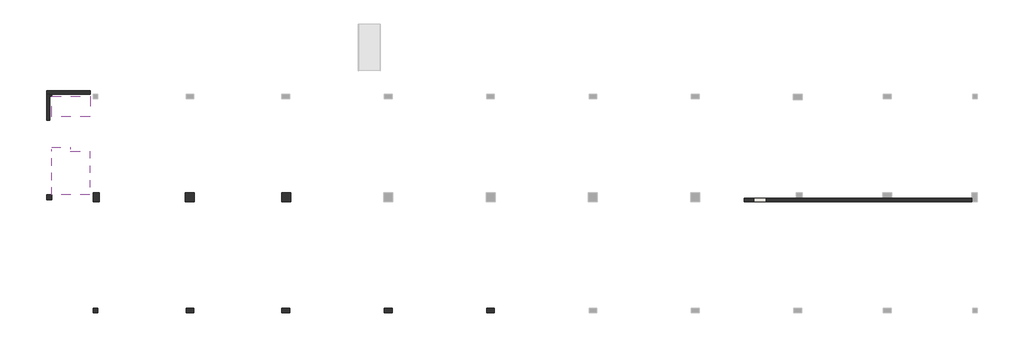
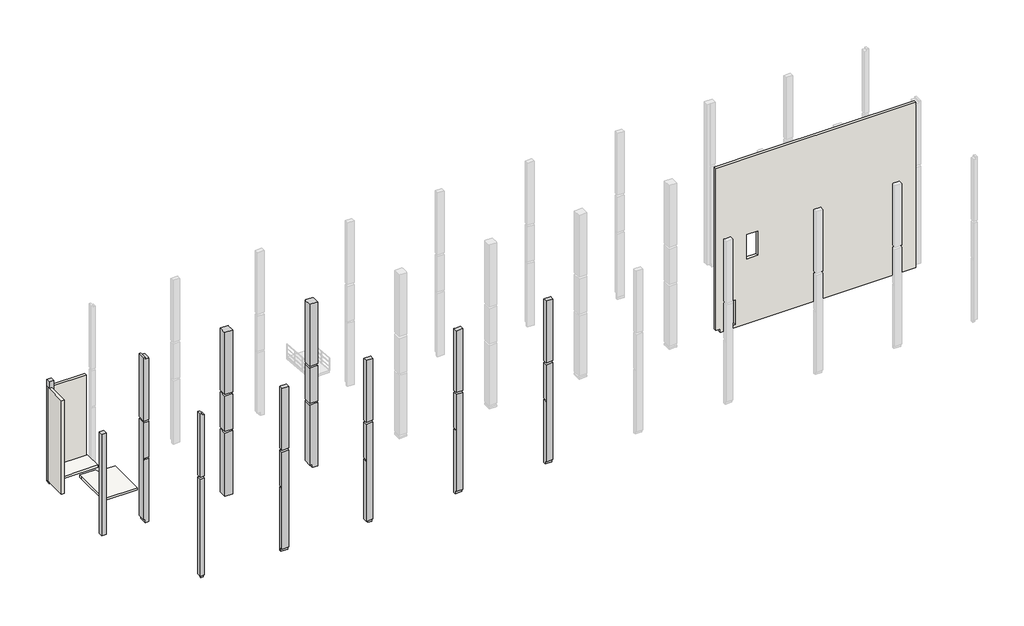
# One storey, part 1 of 3: 10 columns, 3 walls, 2 slabs.
"""IFC4 building model written with IfcOpenShell, lengths in millimetres."""

import ifcopenshell
import ifcopenshell.guid

model = None  # the IFC model being written
_history = None  # IfcOwnerHistory: only IFC2X3 demands one
_inside = {}  # id of a spatial element -> (the spatial element, [elements in it])
_under = {}  # id of a project, library or spatial element -> (it, [spatial elements below it])
_declared = {}  # id of a project -> (the project, [libraries it declares])
_typed = {}  # id of a type object -> (the type object, [elements of that type])
_made_of = {}  # id of a material, layer set ... -> (it, [elements and type objects made of it])


def new_model(schema):
    """Start an empty IFC model of exactly this schema.

    Asked for "IFC4X3", IfcOpenShell would pick the latest addendum, in which some entities
    have other attributes; the version numbers below select the first issue.
    IFC2X3 requires an IfcOwnerHistory on every rooted entity: one is made here for all.
    """
    global model, _history
    if schema == "IFC4X3":
        model = ifcopenshell.file(schema_version=(4, 3, 0, 0))
    else:
        model = ifcopenshell.file(schema=schema)
    _inside.clear()
    _under.clear()
    _declared.clear()
    _typed.clear()
    _made_of.clear()
    _history = None
    if model.schema == "IFC2X3":
        org = make("IfcOrganization", Name="unknown")
        user = make(
            "IfcPersonAndOrganization",
            ThePerson=make("IfcPerson", FamilyName="unknown"),
            TheOrganization=org,
        )
        app = make(
            "IfcApplication",
            ApplicationDeveloper=org,
            Version="unknown",
            ApplicationFullName="unknown",
            ApplicationIdentifier="unknown",
        )
        _history = make(
            "IfcOwnerHistory",
            OwningUser=user,
            OwningApplication=app,
            ChangeAction="ADDED",
            CreationDate=0,
        )
    return model


def make(cls, **values):
    """One entity of the class cls with the attributes given. An attribute that is None is left unset."""
    return model.create_entity(
        cls, **{name: value for name, value in values.items() if value is not None}
    )


def rooted(cls, **values):
    """An entity with a GlobalId (a new one), such as an element, a storey or a relation."""
    return make(cls, GlobalId=ifcopenshell.guid.new(), OwnerHistory=_history, **values)


def si_unit(unit_type, name, prefix=None):
    """IfcSIUnit, for example si_unit("LENGTHUNIT", "METRE", prefix="MILLI")."""
    return make("IfcSIUnit", UnitType=unit_type, Prefix=prefix, Name=name)


def assignment(units):
    """IfcUnitAssignment: the units of a project."""
    return None if units is None else make("IfcUnitAssignment", Units=units)


def point(xyz):
    """IfcCartesianPoint."""
    return None if xyz is None else make("IfcCartesianPoint", Coordinates=xyz)


def direction(xyz):
    """IfcDirection."""
    return None if xyz is None else make("IfcDirection", DirectionRatios=xyz)


def frame(location, z_axis=None, x_axis=None):
    """IfcAxis2Placement3D, a coordinate frame: its origin and axes. An axis left out is left unset."""
    return make(
        "IfcAxis2Placement3D",
        Location=point(location),
        Axis=direction(z_axis),
        RefDirection=direction(x_axis),
    )


def origin():
    """The frame at (0, 0, 0) with its axes left unset."""
    return frame((0.0, 0.0, 0.0))


def place(relative_to, where):
    """IfcLocalPlacement: puts the frame where relative to a parent placement (None: the world)."""
    return make(
        "IfcLocalPlacement", PlacementRelTo=relative_to, RelativePlacement=where
    )


def context(
    kind, dimensions, precision=None, world=None, true_north=None, identifier=None
):
    """IfcGeometricRepresentationContext, for example the 3D "Model" context."""
    return make(
        "IfcGeometricRepresentationContext",
        ContextIdentifier=identifier,
        ContextType=kind,
        CoordinateSpaceDimension=dimensions,
        Precision=precision,
        WorldCoordinateSystem=world,
        TrueNorth=true_north,
    )


def project(units=None, contexts=None):
    """IfcProject with its units and contexts."""
    return rooted(
        "IfcProject",
        Name="project",
        RepresentationContexts=contexts,
        UnitsInContext=assignment(units),
    )


def spatial(cls, under=None, at=None, **own):
    """A site, building, storey or space (cls), placed at a placement, below another one or the project."""
    s = rooted(cls, ObjectPlacement=at, **own)
    if under is not None:
        _under.setdefault(under.id(), (under, []))[1].append(s)
    return s


def polyline(points):
    """IfcPolyline through the points."""
    return make("IfcPolyline", Points=[point(p) for p in points])


def outline(outer, holes=None, kind="AREA"):
    """IfcArbitraryClosedProfileDef: a profile drawn as a closed curve; with holes, ...WithVoids."""
    if holes is None:
        return make("IfcArbitraryClosedProfileDef", ProfileType=kind, OuterCurve=outer)
    return make(
        "IfcArbitraryProfileDefWithVoids",
        ProfileType=kind,
        OuterCurve=outer,
        InnerCurves=holes,
    )


def extrude(swept, where, along, depth):
    """IfcExtrudedAreaSolid: the profile swept, set in the frame where, extruded along a direction by depth."""
    return make(
        "IfcExtrudedAreaSolid",
        SweptArea=swept,
        Position=where,
        ExtrudedDirection=direction(along),
        Depth=depth,
    )


def faces_of(points, faces, orient=None, outer=None):
    """IfcFace entities. A face is a list of loops; a loop is a list of indices into points, from 0.

    orient and outer hold one flag for each loop. By default every Orientation is true, the
    first loop of a face is its IfcFaceOuterBound and the others are IfcFaceBound.
    """
    made = []
    for i, loops in enumerate(faces):
        bounds = []
        for j, loop in enumerate(loops):
            is_outer = j == 0 if outer is None else outer[i][j]
            bounds.append(
                make(
                    "IfcFaceOuterBound" if is_outer else "IfcFaceBound",
                    Bound=make("IfcPolyLoop", Polygon=[points[k] for k in loop]),
                    Orientation=True if orient is None else orient[i][j],
                )
            )
        made.append(make("IfcFace", Bounds=bounds))
    return made


def faceted_brep(points, faces, orient=None, outer=None, voids=None):
    """IfcFacetedBrep: a solid bounded by flat faces; with voids (closed shells), ...WithVoids."""
    shared = [point(p) for p in points]
    hull = make("IfcClosedShell", CfsFaces=faces_of(shared, faces, orient, outer))
    if voids is None:
        return make("IfcFacetedBrep", Outer=hull)
    return make(
        "IfcFacetedBrepWithVoids",
        Outer=hull,
        Voids=[
            make(cls, CfsFaces=faces_of(shared, fs, o, b)) for cls, fs, o, b in voids
        ],
    )


def shape(context_of_items, identifier, shape_type, items):
    """IfcShapeRepresentation: the items that make up one representation, for example the "Body"."""
    return make(
        "IfcShapeRepresentation",
        ContextOfItems=context_of_items,
        RepresentationIdentifier=identifier,
        RepresentationType=shape_type,
        Items=items,
    )


def made_of(thing, what):
    """Note that an element or type object is made of a material, layer set ...; save() writes the relation."""
    if what is not None:
        _made_of.setdefault(what.id(), (what, []))[1].append(thing)
    return thing


def element(
    cls,
    number,
    at=None,
    inside=None,
    cuts=None,
    type_object=None,
    material=None,
    context=None,
    identifier="Body",
    shape_type=None,
    held_by="IfcProductDefinitionShape",
    body=None,
    shapes=None,
    **own,
):
    """One element of the class cls, such as IfcWall. Its Tag is "e" and its number.

    at: its placement. inside: the storey or other place that contains it. cuts: it is an
    opening in that element (IfcRelVoidsElement). A single representation is given by context,
    identifier, shape_type and body (its items); several are given by shapes. held_by: the class
    of the entity that holds the representations. save() writes the other relations.
    """
    e = rooted(cls, Tag="e%d" % number, ObjectPlacement=at, **own)
    if body is not None:
        shapes = [shape(context, identifier, shape_type, body)]
    if shapes is not None:
        e.Representation = make(held_by, Representations=shapes)
    if inside is not None:
        _inside.setdefault(inside.id(), (inside, []))[1].append(e)
    if cuts is not None:
        rooted(
            "IfcRelVoidsElement", RelatingBuildingElement=cuts, RelatedOpeningElement=e
        )
    if type_object is not None:
        _typed.setdefault(type_object.id(), (type_object, []))[1].append(e)
    return made_of(e, material)


def aggregate(whole, parts):
    """IfcRelAggregates: a whole, such as a stair, and the parts it consists of."""
    return rooted("IfcRelAggregates", RelatingObject=whole, RelatedObjects=parts)


def save(model, path):
    """Write the relations noted so far, then the file.

    IfcRelAggregates (storeys below a building ...), IfcRelContainedInSpatialStructure (elements
    in a storey), IfcRelDefinesByType, IfcRelAssociatesMaterial and IfcRelDeclares: one each for
    every whole, place, type object, material and project.
    """
    for whole, parts in _under.values():
        aggregate(whole, parts)
    for where, things in _inside.values():
        rooted(
            "IfcRelContainedInSpatialStructure",
            RelatedElements=things,
            RelatingStructure=where,
        )
    for kind, things in _typed.values():
        rooted("IfcRelDefinesByType", RelatedObjects=things, RelatingType=kind)
    for what, things in _made_of.values():
        rooted("IfcRelAssociatesMaterial", RelatedObjects=things, RelatingMaterial=what)
    for by, libraries in _declared.values():
        rooted("IfcRelDeclares", RelatingContext=by, RelatedDefinitions=libraries)
    model.write(path)


model = new_model("IFC4")

# Units and contexts
model_context = context("Model", 3, world=origin())
ifc_project = project(units=[si_unit("LENGTHUNIT", "METRE", prefix="MILLI")], contexts=[model_context])

# Site, building, storey
site = spatial("IfcSite", under=ifc_project)
building = spatial("IfcBuilding", under=site)
storey = spatial("IfcBuildingStorey", under=building, Name="G.L", Elevation=-150.0381366)

# Columns
placement = place(None, origin())
element("IfcColumn", 1, ObjectType="RC_Column_Rectangular : H_SC_AR_S15_AG_W700xL700_C1", at=placement, inside=storey, context=model_context, shape_type="Brep", body=[
    faceted_brep([(400.0, 9849.5208589, -150.0381366), (400.0, 9149.5208589, -150.0381366), (100.0, 9149.5208589, -150.0381366), (100.0, 9849.5208589, -150.0381366), (0.0, 9849.5208589, 5799.9618634), (0.0, 9149.5208589, 5799.9618634), (100.0, 9149.5208589, 5799.9618634), (400.0, 9149.5208589, 5799.9618634), (400.0, 9199.5208589, 5799.9618634), (400.0, 9799.5208589, 5799.9618634), (400.0, 9849.5208589, 5799.9618634), (150.0, 9849.5208589, 5799.9618634), (100.0, 9849.5208589, 5799.9618634), (0.0, 9149.5208589, 5949.9618634), (0.0, 9849.5208589, 5949.9618634), (400.0, 9849.5208589, 5949.9618634), (400.0, 9149.5208589, 5949.9618634), (0.0, 9849.5208589, 5899.9618634), (400.0, 9149.5208589, 9269.9618634), (400.0, 9199.5208589, 9269.9618634), (400.0, 9799.5208589, 9269.9618634), (400.0, 9849.5208589, 9269.9618634), (100.0, 9849.5208589, 9269.9618634), (-50.0, 9849.5208589, 9269.9618634), (-50.0, 9149.5208589, 9269.9618634), (100.0, 9149.5208589, 9269.9618634), (100.0, 9149.5208589, 149.9618634), (100.0, 9849.5208589, 149.9618634), (-50.0, 9149.5208589, 149.9618634), (-50.0, 9849.5208589, 149.9618634), (-50.0, 9149.5208589, 5249.9618634), (-50.0, 9149.5208589, 5949.9618634), (-50.0, 9149.5208589, 8749.9618634), (-50.0, 9849.5208589, 8749.9618634), (-50.0, 9849.5208589, 5949.9618634), (-50.0, 9849.5208589, 5899.9618634), (-50.0, 9849.5208589, 5199.9618634)], [[[0, 1, 2, 3]], [[4, 5, 6, 7, 8, 9, 10, 11, 12]], [[13, 14, 15, 16]], [[5, 4, 17, 14, 13]], [[1, 0, 10, 9, 8, 7]], [[18, 19, 20, 21, 22, 23, 24, 25]], [[16, 15, 21, 20, 19, 18]], [[26, 27, 3, 2]], [[27, 26, 28, 29]], [[28, 30, 31, 32, 24, 23, 33, 34, 35, 36, 29]], [[1, 7, 6, 5, 13, 16, 18, 25, 24, 32, 31, 30, 28, 26, 2]], [[10, 0, 3, 27, 29, 36, 35, 34, 33, 23, 22, 21, 15, 14, 17, 4, 12, 11]]]),
    faceted_brep([(400.0, 9149.5208589, 9449.9618634), (400.0, 9849.5208589, 9449.9618634), (400.0, 9849.5208589, 15259.9618634), (400.0, 9724.5208589, 15259.9618634), (400.0, 9274.5208589, 15259.9618634), (400.0, 9149.5208589, 15259.9618634), (-50.0, 9149.5208589, 9449.9618634), (100.0, 9149.5208589, 15259.9618634), (100.0, 9149.5208589, 15409.9618634), (-50.0, 9149.5208589, 15409.9618634), (-50.0, 9149.5208589, 14709.9618634), (-50.0, 9849.5208589, 9449.9618634), (-50.0, 9849.5208589, 14709.9618634), (-50.0, 9849.5208589, 15409.9618634), (100.0, 9849.5208589, 15409.9618634), (100.0, 9849.5208589, 15259.9618634)], [[[0, 1, 2, 3, 4, 5]], [[6, 0, 5, 7, 8, 9, 10]], [[1, 11, 12, 13, 14, 15, 2]], [[8, 14, 13, 9]], [[1, 0, 6, 11]], [[15, 7, 5, 4, 3, 2]], [[7, 15, 14, 8]], [[6, 10, 9, 13, 12, 11]]]),
])
element("IfcColumn", 2, ObjectType="RC_Column_Rectangular : H_SC_AR_S15_AG_W700xL700_C1", at=placement, inside=storey, context=model_context, shape_type="Brep", body=[
    faceted_brep([(7850.0, 9849.5208589, -150.0381366), (7850.0, 9149.5208589, -150.0381366), (7150.0, 9149.5208589, -150.0381366), (7150.0, 9849.5208589, -150.0381366), (7850.0, 9149.5208589, 5799.9618634), (7850.0, 9199.5208589, 5799.9618634), (7850.0, 9799.5208589, 5799.9618634), (7850.0, 9849.5208589, 5799.9618634), (7750.0, 9849.5208589, 5799.9618634), (7250.0, 9849.5208589, 5799.9618634), (7150.0, 9849.5208589, 5799.9618634), (7150.0, 9799.5208589, 5799.9618634), (7150.0, 9199.5208589, 5799.9618634), (7150.0, 9149.5208589, 5799.9618634), (7250.0, 9149.5208589, 5799.9618634), (7750.0, 9149.5208589, 5799.9618634)], [[[0, 1, 2, 3]], [[4, 5, 6, 7, 8, 9, 10, 11, 12, 13, 14, 15]], [[1, 0, 7, 6, 5, 4]], [[2, 1, 4, 15, 14, 13]], [[3, 2, 13, 12, 11, 10]], [[0, 3, 10, 9, 8, 7]]]),
    faceted_brep([(7850.0, 9149.5208589, 9449.9618634), (7850.0, 9849.5208589, 9449.9618634), (7850.0, 9849.5208589, 15259.9618634), (7850.0, 9724.5208589, 15259.9618634), (7850.0, 9274.5208589, 15259.9618634), (7850.0, 9149.5208589, 15259.9618634), (7150.0, 9149.5208589, 9449.9618634), (7725.0, 9149.5208589, 15259.9618634), (7275.0, 9149.5208589, 15259.9618634), (7150.0, 9149.5208589, 15259.9618634), (7150.0, 9849.5208589, 9449.9618634), (7150.0, 9274.5208589, 15259.9618634), (7150.0, 9724.5208589, 15259.9618634), (7150.0, 9849.5208589, 15259.9618634), (7275.0, 9849.5208589, 15259.9618634), (7725.0, 9849.5208589, 15259.9618634)], [[[0, 1, 2, 3, 4, 5]], [[6, 0, 5, 7, 8, 9]], [[10, 6, 9, 11, 12, 13]], [[1, 10, 13, 14, 15, 2]], [[1, 0, 6, 10]], [[5, 4, 3, 2, 15, 14, 13, 12, 11, 9, 8, 7]]]),
    faceted_brep([(7850.0, 9849.5208589, 5949.9618634), (7850.0, 9149.5208589, 5949.9618634), (7150.0, 9149.5208589, 5949.9618634), (7150.0, 9849.5208589, 5949.9618634), (7850.0, 9149.5208589, 9269.9618634), (7850.0, 9199.5208589, 9269.9618634), (7850.0, 9799.5208589, 9269.9618634), (7850.0, 9849.5208589, 9269.9618634), (7750.0, 9849.5208589, 9269.9618634), (7250.0, 9849.5208589, 9269.9618634), (7150.0, 9849.5208589, 9269.9618634), (7150.0, 9799.5208589, 9269.9618634), (7150.0, 9199.5208589, 9269.9618634), (7150.0, 9149.5208589, 9269.9618634), (7250.0, 9149.5208589, 9269.9618634), (7750.0, 9149.5208589, 9269.9618634)], [[[0, 1, 2, 3]], [[4, 5, 6, 7, 8, 9, 10, 11, 12, 13, 14, 15]], [[1, 0, 7, 6, 5, 4]], [[2, 1, 4, 15, 14, 13]], [[3, 2, 13, 12, 11, 10]], [[0, 3, 10, 9, 8, 7]]]),
])
element("IfcColumn", 3, ObjectType="RC_Column_Rectangular : H_SC_AR_S15_AG_W700xL700_C1", at=placement, inside=storey, context=model_context, shape_type="Brep", body=[
    faceted_brep([(15400.0, 9849.5208589, -150.0381366), (15400.0, 9149.5208589, -150.0381366), (14950.0, 9149.5208589, -150.0381366), (14950.0, 9849.5208589, -150.0381366), (15400.0, 9149.5208589, 5799.9618634), (15400.0, 9199.5208589, 5799.9618634), (15400.0, 9799.5208589, 5799.9618634), (15400.0, 9849.5208589, 5799.9618634), (15250.0, 9849.5208589, 5799.9618634), (14750.0, 9849.5208589, 5799.9618634), (14700.0, 9849.5208589, 5799.9618634), (14700.0, 9799.5208589, 5799.9618634), (14700.0, 9199.5208589, 5799.9618634), (14700.0, 9149.5208589, 5799.9618634), (14750.0, 9149.5208589, 5799.9618634), (15250.0, 9149.5208589, 5799.9618634), (15400.0, 9849.5208589, -0.0381366), (15400.0, 9849.5208589, 149.9618634), (15400.0, 9149.5208589, 149.9618634), (15400.0, 9149.5208589, -0.0381366), (14700.0, 9149.5208589, 149.9618634), (14950.0, 9149.5208589, 149.9618634), (14950.0, 9149.5208589, -0.0381366), (14700.0, 9849.5208589, 149.9618634), (14950.0, 9849.5208589, -0.0381366), (14950.0, 9849.5208589, 149.9618634)], [[[0, 1, 2, 3]], [[4, 5, 6, 7, 8, 9, 10, 11, 12, 13, 14, 15]], [[1, 0, 16, 17, 7, 6, 5, 4, 18, 19]], [[1, 19, 18, 4, 15, 14, 13, 20, 21, 22, 2]], [[13, 12, 11, 10, 23, 20]], [[16, 0, 3, 24, 25, 23, 10, 9, 8, 7, 17]], [[21, 25, 24, 3, 2, 22]], [[25, 21, 20, 23]]]),
    faceted_brep([(15400.0, 9149.5208589, 9449.9618634), (15400.0, 9849.5208589, 9449.9618634), (15400.0, 9849.5208589, 15259.9618634), (15400.0, 9724.5208589, 15259.9618634), (15400.0, 9274.5208589, 15259.9618634), (15400.0, 9149.5208589, 15259.9618634), (14700.0, 9149.5208589, 9449.9618634), (15225.0, 9149.5208589, 15259.9618634), (14775.0, 9149.5208589, 15259.9618634), (14700.0, 9149.5208589, 15259.9618634), (14700.0, 9849.5208589, 9449.9618634), (14700.0, 9274.5208589, 15259.9618634), (14700.0, 9724.5208589, 15259.9618634), (14700.0, 9849.5208589, 15259.9618634), (14775.0, 9849.5208589, 15259.9618634), (15225.0, 9849.5208589, 15259.9618634)], [[[0, 1, 2, 3, 4, 5]], [[6, 0, 5, 7, 8, 9]], [[10, 6, 9, 11, 12, 13]], [[1, 10, 13, 14, 15, 2]], [[1, 0, 6, 10]], [[5, 4, 3, 2, 15, 14, 13, 12, 11, 9, 8, 7]]]),
    faceted_brep([(15400.0, 9849.5208589, 5949.9618634), (15400.0, 9149.5208589, 5949.9618634), (14700.0, 9149.5208589, 5949.9618634), (14700.0, 9849.5208589, 5949.9618634), (15400.0, 9149.5208589, 9269.9618634), (15400.0, 9199.5208589, 9269.9618634), (15400.0, 9799.5208589, 9269.9618634), (15400.0, 9849.5208589, 9269.9618634), (15250.0, 9849.5208589, 9269.9618634), (14750.0, 9849.5208589, 9269.9618634), (14700.0, 9849.5208589, 9269.9618634), (14700.0, 9799.5208589, 9269.9618634), (14700.0, 9199.5208589, 9269.9618634), (14700.0, 9149.5208589, 9269.9618634), (14750.0, 9149.5208589, 9269.9618634), (15250.0, 9149.5208589, 9269.9618634)], [[[0, 1, 2, 3]], [[4, 5, 6, 7, 8, 9, 10, 11, 12, 13, 14, 15]], [[1, 0, 7, 6, 5, 4]], [[2, 1, 4, 15, 14, 13]], [[3, 2, 13, 12, 11, 10]], [[0, 3, 10, 9, 8, 7]]]),
])
element("IfcColumn", 4, ObjectType="RC_Column_Rectangular : H_SC_AR_S15_AG_W600xL600_C2", at=placement, inside=storey, context=model_context, shape_type="Brep", body=[
    faceted_brep([(30700.0, 799.5208589, -150.0381366), (31300.0, 799.5208589, -150.0381366), (31300.0, 599.5208589, -150.0381366), (30700.0, 599.5208589, -150.0381366), (30700.0, 499.5208589, 5799.9618634), (31300.0, 499.5208589, 5799.9618634), (31300.0, 599.5208589, 5799.9618634), (31300.0, 799.5208589, 5799.9618634), (31250.0, 799.5208589, 5799.9618634), (30750.0, 799.5208589, 5799.9618634), (30700.0, 799.5208589, 5799.9618634), (30700.0, 599.5208589, 5799.9618634), (31300.0, 499.5208589, 5949.9618634), (30700.0, 499.5208589, 5949.9618634), (30700.0, 799.5208589, 5949.9618634), (31300.0, 799.5208589, 5949.9618634), (30700.0, 799.5208589, -0.0381366), (30700.0, 799.5208589, 149.9618634), (31300.0, 799.5208589, 149.9618634), (31300.0, 799.5208589, -0.0381366), (31300.0, 449.5208589, 9269.9618634), (31300.0, 599.5208589, 9269.9618634), (31300.0, 799.5208589, 9269.9618634), (31250.0, 799.5208589, 9269.9618634), (30750.0, 799.5208589, 9269.9618634), (30700.0, 799.5208589, 9269.9618634), (30700.0, 599.5208589, 9269.9618634), (30700.0, 449.5208589, 9269.9618634), (31300.0, 599.5208589, 149.9618634), (30700.0, 599.5208589, 149.9618634), (31300.0, 449.5208589, 149.9618634), (30700.0, 449.5208589, 149.9618634), (31300.0, 449.5208589, 5249.9618634), (31300.0, 449.5208589, 5949.9618634), (31300.0, 449.5208589, 8749.9618634), (30700.0, 449.5208589, 8749.9618634), (30700.0, 449.5208589, 5949.9618634), (30700.0, 449.5208589, 5249.9618634)], [[[0, 1, 2, 3]], [[4, 5, 6, 7, 8, 9, 10, 11]], [[12, 13, 14, 15]], [[5, 4, 13, 12]], [[1, 0, 16, 17, 10, 9, 8, 7, 18, 19]], [[20, 21, 22, 23, 24, 25, 26, 27]], [[15, 14, 25, 24, 23, 22]], [[28, 29, 3, 2]], [[29, 28, 30, 31]], [[30, 32, 33, 34, 20, 27, 35, 36, 37, 31]], [[1, 19, 18, 7, 6, 5, 12, 15, 22, 21, 20, 34, 33, 32, 30, 28, 2]], [[16, 0, 3, 29, 31, 37, 36, 35, 27, 26, 25, 14, 13, 4, 11, 10, 17]]]),
    faceted_brep([(31300.0, 449.5208589, 9449.9618634), (31300.0, 799.5208589, 9449.9618634), (31300.0, 799.5208589, 15259.9618634), (31300.0, 599.5208589, 15259.9618634), (31300.0, 449.5208589, 15259.9618634), (31300.0, 449.5208589, 14709.9618634), (30700.0, 799.5208589, 9449.9618634), (30700.0, 449.5208589, 9449.9618634), (30700.0, 449.5208589, 14709.9618634), (30700.0, 449.5208589, 15259.9618634), (30700.0, 599.5208589, 15259.9618634), (30700.0, 799.5208589, 15259.9618634), (30775.0, 799.5208589, 15259.9618634), (31225.0, 799.5208589, 15259.9618634)], [[[0, 1, 2, 3, 4, 5]], [[6, 7, 8, 9, 10, 11]], [[1, 6, 11, 12, 13, 2]], [[1, 0, 7, 6]], [[4, 3, 2, 13, 12, 11, 10, 9]], [[0, 5, 4, 9, 8, 7]]]),
])
element("IfcColumn", 5, ObjectType="RC_Column_Rectangular : H_SC_AR_S15_AG_W600xL600_C2", at=placement, inside=storey, context=model_context, shape_type="Brep", body=[
    faceted_brep([(22700.0, 799.5208589, -150.0381366), (23300.0, 799.5208589, -150.0381366), (23300.0, 599.5208589, -150.0381366), (22700.0, 599.5208589, -150.0381366), (22700.0, 499.5208589, 5799.9618634), (23300.0, 499.5208589, 5799.9618634), (23300.0, 599.5208589, 5799.9618634), (23300.0, 799.5208589, 5799.9618634), (23250.0, 799.5208589, 5799.9618634), (22750.0, 799.5208589, 5799.9618634), (22700.0, 799.5208589, 5799.9618634), (22700.0, 599.5208589, 5799.9618634), (23300.0, 499.5208589, 5949.9618634), (22700.0, 499.5208589, 5949.9618634), (22700.0, 799.5208589, 5949.9618634), (23300.0, 799.5208589, 5949.9618634), (22700.0, 799.5208589, -0.0381366), (22700.0, 799.5208589, 149.9618634), (23300.0, 799.5208589, 149.9618634), (23300.0, 799.5208589, -0.0381366), (23300.0, 449.5208589, 9269.9618634), (23300.0, 599.5208589, 9269.9618634), (23300.0, 799.5208589, 9269.9618634), (23250.0, 799.5208589, 9269.9618634), (22750.0, 799.5208589, 9269.9618634), (22700.0, 799.5208589, 9269.9618634), (22700.0, 599.5208589, 9269.9618634), (22700.0, 449.5208589, 9269.9618634), (23300.0, 599.5208589, 149.9618634), (22700.0, 599.5208589, 149.9618634), (23300.0, 449.5208589, 149.9618634), (22700.0, 449.5208589, 149.9618634), (23300.0, 449.5208589, 5249.9618634), (23300.0, 449.5208589, 5949.9618634), (23300.0, 449.5208589, 8749.9618634), (22700.0, 449.5208589, 8749.9618634), (22700.0, 449.5208589, 5949.9618634), (22700.0, 449.5208589, 5249.9618634)], [[[0, 1, 2, 3]], [[4, 5, 6, 7, 8, 9, 10, 11]], [[12, 13, 14, 15]], [[5, 4, 13, 12]], [[1, 0, 16, 17, 10, 9, 8, 7, 18, 19]], [[20, 21, 22, 23, 24, 25, 26, 27]], [[15, 14, 25, 24, 23, 22]], [[28, 29, 3, 2]], [[29, 28, 30, 31]], [[30, 32, 33, 34, 20, 27, 35, 36, 37, 31]], [[1, 19, 18, 7, 6, 5, 12, 15, 22, 21, 20, 34, 33, 32, 30, 28, 2]], [[16, 0, 3, 29, 31, 37, 36, 35, 27, 26, 25, 14, 13, 4, 11, 10, 17]]]),
    faceted_brep([(23300.0, 449.5208589, 9449.9618634), (23300.0, 799.5208589, 9449.9618634), (23300.0, 799.5208589, 15259.9618634), (23300.0, 599.5208589, 15259.9618634), (23300.0, 449.5208589, 15259.9618634), (23300.0, 449.5208589, 14709.9618634), (22700.0, 799.5208589, 9449.9618634), (22700.0, 449.5208589, 9449.9618634), (22700.0, 449.5208589, 14709.9618634), (22700.0, 449.5208589, 15259.9618634), (22700.0, 599.5208589, 15259.9618634), (22700.0, 799.5208589, 15259.9618634), (22775.0, 799.5208589, 15259.9618634), (23225.0, 799.5208589, 15259.9618634)], [[[0, 1, 2, 3, 4, 5]], [[6, 7, 8, 9, 10, 11]], [[1, 6, 11, 12, 13, 2]], [[1, 0, 7, 6]], [[4, 3, 2, 13, 12, 11, 10, 9]], [[0, 5, 4, 9, 8, 7]]]),
])
element("IfcColumn", 6, ObjectType="RC_Column_Rectangular : H_SC_AR_S15_AG_W600xL600_C2", at=placement, inside=storey, context=model_context, shape_type="Brep", body=[
    faceted_brep([(15300.0, 799.5208589, -150.0381366), (15300.0, 599.5208589, -150.0381366), (14950.0, 599.5208589, -150.0381366), (14950.0, 799.5208589, -150.0381366), (14700.0, 499.5208589, 5799.9618634), (15300.0, 499.5208589, 5799.9618634), (15300.0, 599.5208589, 5799.9618634), (15300.0, 799.5208589, 5799.9618634), (15250.0, 799.5208589, 5799.9618634), (14750.0, 799.5208589, 5799.9618634), (14700.0, 799.5208589, 5799.9618634), (14700.0, 599.5208589, 5799.9618634), (15300.0, 499.5208589, 5949.9618634), (14700.0, 499.5208589, 5949.9618634), (14700.0, 799.5208589, 5949.9618634), (15300.0, 799.5208589, 5949.9618634), (15300.0, 799.5208589, -0.0381366), (14950.0, 799.5208589, 149.9618634), (14700.0, 799.5208589, 149.9618634), (15300.0, 799.5208589, 149.9618634), (15300.0, 449.5208589, 9269.9618634), (15300.0, 599.5208589, 9269.9618634), (15300.0, 799.5208589, 9269.9618634), (15250.0, 799.5208589, 9269.9618634), (14750.0, 799.5208589, 9269.9618634), (14700.0, 799.5208589, 9269.9618634), (14700.0, 599.5208589, 9269.9618634), (14700.0, 449.5208589, 9269.9618634), (15300.0, 599.5208589, 149.9618634), (14950.0, 599.5208589, 149.9618634), (15300.0, 449.5208589, 149.9618634), (14700.0, 449.5208589, 149.9618634), (14700.0, 599.5208589, 149.9618634), (15300.0, 449.5208589, 5249.9618634), (15300.0, 449.5208589, 5949.9618634), (15300.0, 449.5208589, 8749.9618634), (14700.0, 449.5208589, 8749.9618634), (14700.0, 449.5208589, 5949.9618634), (14700.0, 449.5208589, 5249.9618634)], [[[0, 1, 2, 3]], [[4, 5, 6, 7, 8, 9, 10, 11]], [[12, 13, 14, 15]], [[5, 4, 13, 12]], [[16, 0, 3, 17, 18, 10, 9, 8, 7, 19]], [[20, 21, 22, 23, 24, 25, 26, 27]], [[15, 14, 25, 24, 23, 22]], [[1, 28, 29, 2]], [[18, 17, 29, 28, 30, 31, 32]], [[30, 33, 34, 35, 20, 27, 36, 37, 38, 31]], [[0, 16, 19, 7, 6, 5, 12, 15, 22, 21, 20, 35, 34, 33, 30, 28, 1]], [[4, 11, 10, 18, 32, 31, 38, 37, 36, 27, 26, 25, 14, 13]], [[29, 17, 3, 2]]]),
    faceted_brep([(15300.0, 449.5208589, 9449.9618634), (15300.0, 799.5208589, 9449.9618634), (15300.0, 799.5208589, 15259.9618634), (15300.0, 599.5208589, 15259.9618634), (15300.0, 449.5208589, 15259.9618634), (15300.0, 449.5208589, 14709.9618634), (14700.0, 799.5208589, 9449.9618634), (14700.0, 449.5208589, 9449.9618634), (14700.0, 449.5208589, 14709.9618634), (14700.0, 449.5208589, 15259.9618634), (14700.0, 599.5208589, 15259.9618634), (14700.0, 799.5208589, 15259.9618634), (14775.0, 799.5208589, 15259.9618634), (15225.0, 799.5208589, 15259.9618634)], [[[0, 1, 2, 3, 4, 5]], [[6, 7, 8, 9, 10, 11]], [[1, 6, 11, 12, 13, 2]], [[1, 0, 7, 6]], [[4, 3, 2, 13, 12, 11, 10, 9]], [[0, 5, 4, 9, 8, 7]]]),
])
element("IfcColumn", 7, ObjectType="RC_Column_Rectangular : H_SC_AR_S15_AG_W600xL600_C2", at=placement, inside=storey, context=model_context, shape_type="Brep", body=[
    faceted_brep([(7200.0, 799.5208589, -150.0381366), (7800.0, 799.5208589, -150.0381366), (7800.0, 599.5208589, -150.0381366), (7200.0, 599.5208589, -150.0381366), (7200.0, 499.5208589, 5799.9618634), (7800.0, 499.5208589, 5799.9618634), (7800.0, 599.5208589, 5799.9618634), (7800.0, 799.5208589, 5799.9618634), (7750.0, 799.5208589, 5799.9618634), (7250.0, 799.5208589, 5799.9618634), (7200.0, 799.5208589, 5799.9618634), (7200.0, 599.5208589, 5799.9618634), (7800.0, 499.5208589, 5949.9618634), (7200.0, 499.5208589, 5949.9618634), (7200.0, 799.5208589, 5949.9618634), (7800.0, 799.5208589, 5949.9618634), (7800.0, 449.5208589, 9269.9618634), (7800.0, 599.5208589, 9269.9618634), (7800.0, 799.5208589, 9269.9618634), (7750.0, 799.5208589, 9269.9618634), (7250.0, 799.5208589, 9269.9618634), (7200.0, 799.5208589, 9269.9618634), (7200.0, 599.5208589, 9269.9618634), (7200.0, 449.5208589, 9269.9618634), (7800.0, 599.5208589, 149.9618634), (7200.0, 599.5208589, 149.9618634), (7800.0, 449.5208589, 149.9618634), (7200.0, 449.5208589, 149.9618634), (7800.0, 449.5208589, 5249.9618634), (7800.0, 449.5208589, 5949.9618634), (7800.0, 449.5208589, 8749.9618634), (7200.0, 449.5208589, 8749.9618634), (7200.0, 449.5208589, 5949.9618634), (7200.0, 449.5208589, 5249.9618634)], [[[0, 1, 2, 3]], [[4, 5, 6, 7, 8, 9, 10, 11]], [[12, 13, 14, 15]], [[5, 4, 13, 12]], [[1, 0, 10, 9, 8, 7]], [[16, 17, 18, 19, 20, 21, 22, 23]], [[15, 14, 21, 20, 19, 18]], [[24, 25, 3, 2]], [[25, 24, 26, 27]], [[26, 28, 29, 30, 16, 23, 31, 32, 33, 27]], [[1, 7, 6, 5, 12, 15, 18, 17, 16, 30, 29, 28, 26, 24, 2]], [[10, 0, 3, 25, 27, 33, 32, 31, 23, 22, 21, 14, 13, 4, 11]]]),
    faceted_brep([(7800.0, 449.5208589, 9449.9618634), (7800.0, 799.5208589, 9449.9618634), (7800.0, 799.5208589, 15259.9618634), (7800.0, 599.5208589, 15259.9618634), (7800.0, 449.5208589, 15259.9618634), (7800.0, 449.5208589, 14709.9618634), (7200.0, 799.5208589, 9449.9618634), (7200.0, 449.5208589, 9449.9618634), (7200.0, 449.5208589, 14709.9618634), (7200.0, 449.5208589, 15259.9618634), (7200.0, 599.5208589, 15259.9618634), (7200.0, 799.5208589, 15259.9618634), (7275.0, 799.5208589, 15259.9618634), (7725.0, 799.5208589, 15259.9618634)], [[[0, 1, 2, 3, 4, 5]], [[6, 7, 8, 9, 10, 11]], [[1, 6, 11, 12, 13, 2]], [[1, 0, 7, 6]], [[4, 3, 2, 13, 12, 11, 10, 9]], [[0, 5, 4, 9, 8, 7]]]),
])
element("IfcColumn", 8, ObjectType="RC_Column_Rectangular : H_SC_AR_S15_AG_W600xL600_C2", at=placement, inside=storey, context=model_context, shape_type="Brep", body=[
    faceted_brep([(300.0, 799.5208589, -150.0381366), (300.0, 599.5208589, -150.0381366), (100.0, 599.5208589, -150.0381366), (100.0, 799.5208589, -150.0381366), (0.0, 799.5208589, 5799.9618634), (0.0, 499.5208589, 5799.9618634), (300.0, 499.5208589, 5799.9618634), (300.0, 599.5208589, 5799.9618634), (300.0, 799.5208589, 5799.9618634), (100.0, 799.5208589, 5799.9618634), (300.0, 499.5208589, 5949.9618634), (0.0, 499.5208589, 5949.9618634), (0.0, 799.5208589, 5949.9618634), (300.0, 799.5208589, 5949.9618634), (300.0, 449.5208589, 9269.9618634), (300.0, 599.5208589, 9269.9618634), (300.0, 799.5208589, 9269.9618634), (100.0, 799.5208589, 9269.9618634), (-50.0, 799.5208589, 9269.9618634), (-50.0, 449.5208589, 9269.9618634), (300.0, 599.5208589, 149.9618634), (100.0, 599.5208589, 149.9618634), (300.0, 449.5208589, 149.9618634), (100.0, 449.5208589, 149.9618634), (-50.0, 449.5208589, 149.9618634), (-50.0, 799.5208589, 149.9618634), (100.0, 799.5208589, 149.9618634), (-50.0, 799.5208589, 8749.9618634), (-50.0, 799.5208589, 5949.9618634), (-50.0, 799.5208589, 5249.9618634), (300.0, 449.5208589, 5249.9618634), (300.0, 449.5208589, 5949.9618634), (300.0, 449.5208589, 8749.9618634)], [[[0, 1, 2, 3]], [[4, 5, 6, 7, 8, 9]], [[10, 11, 12, 13]], [[5, 11, 10, 6]], [[11, 5, 4, 12]], [[14, 15, 16, 17, 18, 19]], [[1, 20, 21, 2]], [[21, 20, 22, 23, 24, 25, 26]], [[21, 26, 3, 2]], [[18, 27, 28, 29, 25, 24, 19]], [[8, 0, 3, 26, 25, 29, 28, 27, 18, 17, 16, 13, 12, 4, 9]], [[22, 30, 31, 32, 14, 19, 24, 23]], [[0, 8, 7, 6, 10, 13, 16, 15, 14, 32, 31, 30, 22, 20, 1]]]),
    faceted_brep([(300.0, 449.5208589, 9449.9618634), (300.0, 799.5208589, 9449.9618634), (300.0, 799.5208589, 15259.9618634), (300.0, 599.5208589, 15259.9618634), (300.0, 449.5208589, 15259.9618634), (300.0, 449.5208589, 14709.9618634), (-50.0, 799.5208589, 9449.9618634), (-50.0, 799.5208589, 14709.9618634), (-50.0, 799.5208589, 15409.9618634), (100.0, 799.5208589, 15409.9618634), (100.0, 799.5208589, 15259.9618634), (100.0, 449.5208589, 15409.9618634), (-50.0, 449.5208589, 15409.9618634), (-50.0, 449.5208589, 9449.9618634), (100.0, 449.5208589, 15259.9618634)], [[[0, 1, 2, 3, 4, 5]], [[1, 6, 7, 8, 9, 10, 2]], [[11, 9, 8, 12]], [[1, 0, 13, 6]], [[10, 14, 4, 3, 2]], [[14, 10, 9, 11]], [[8, 7, 6, 13, 12]], [[0, 5, 4, 14, 11, 12, 13]]]),
])
element("IfcColumn", 9, ObjectType="RC_Column_Rectangular : H_SC_AR_S15_AG_W400xL400_C3", at=placement, inside=storey, context=model_context, shape_type="Brep", body=[
    faceted_brep([(-3300.0, 17799.5208589, -150.0381366), (-3300.0, 17399.5208589, -150.0381366), (-3700.0, 17399.5208589, -150.0381366), (-3700.0, 17799.5208589, -150.0381366), (-3300.0, 17799.5208589, -20.0381366), (-3300.0, 17549.5208589, -20.0381366), (-3300.0, 17549.5208589, 2339.9618634), (-3300.0, 17549.5208589, 2939.9618634), (-3300.0, 17549.5208589, 5299.9618634), (-3300.0, 17549.5208589, 5899.9618634), (-3300.0, 17549.5208589, 8799.9618634), (-3300.0, 17799.5208589, 8799.9618634), (-3300.0, 17799.5208589, 9399.9618634), (-3300.0, 17399.5208589, 9399.9618634), (-3300.0, 17399.5208589, 8799.9618634), (-3300.0, 17399.5208589, 5899.9618634), (-3300.0, 17399.5208589, 5299.9618634), (-3300.0, 17399.5208589, 2939.9618634), (-3300.0, 17399.5208589, 2339.9618634), (-3300.0, 17399.5208589, -20.0381366), (-3700.0, 17399.5208589, 9399.9618634), (-3700.0, 17399.5208589, 8799.9618634), (-3450.0, 17399.5208589, 8799.9618634), (-3450.0, 17399.5208589, 5899.9618634), (-3450.0, 17399.5208589, 5299.9618634), (-3450.0, 17399.5208589, 2939.9618634), (-3450.0, 17399.5208589, 2339.9618634), (-3450.0, 17399.5208589, -20.0381366), (-3700.0, 17399.5208589, -20.0381366), (-3700.0, 17799.5208589, 9399.9618634), (-3700.0, 17799.5208589, 8799.9618634), (-3700.0, 17549.5208589, 8799.9618634), (-3450.0, 17549.5208589, -20.0381366), (-3450.0, 17549.5208589, 8799.9618634), (-3700.0, 17799.5208589, -20.0381366), (-3700.0, 17549.5208589, -20.0381366)], [[[0, 1, 2, 3]], [[1, 0, 4, 5, 6, 7, 8, 9, 10, 11, 12, 13, 14, 15, 16, 17, 18, 19]], [[2, 1, 19, 18, 17, 16, 15, 14, 13, 20, 21, 22, 23, 24, 25, 26, 27, 28]], [[20, 29, 30, 31, 21]], [[29, 12, 11, 30]], [[13, 12, 29, 20]], [[32, 27, 26, 25, 24, 23, 22, 33]], [[27, 32, 5, 4, 34, 35, 28]], [[33, 22, 21, 31, 30, 11, 10]], [[5, 32, 33, 10, 9, 8, 7, 6]], [[3, 2, 28, 35, 34]], [[0, 3, 34, 4]]]),
])
element("IfcColumn", 10, ObjectType="RC_Column_Rectangular : H_SC_AR_S15_AG_W400xL400_C3", at=placement, inside=storey, context=model_context, shape_type="Brep", body=[
    faceted_brep([(-3300.0, 9699.5208589, -150.0381366), (-3300.0, 9299.5208589, -150.0381366), (-3700.0, 9299.5208589, -150.0381366), (-3700.0, 9699.5208589, -150.0381366), (-3300.0, 9699.5208589, 9399.9618634), (-3300.0, 9299.5208589, 9399.9618634), (-3300.0, 9299.5208589, 8799.9618634), (-3300.0, 9299.5208589, 5899.9618634), (-3300.0, 9299.5208589, 5299.9618634), (-3300.0, 9299.5208589, 2939.9618634), (-3300.0, 9299.5208589, 2339.9618634), (-3300.0, 9299.5208589, -20.0381366), (-3300.0, 9699.5208589, -20.0381366), (-3300.0, 9699.5208589, 2339.9618634), (-3300.0, 9699.5208589, 2939.9618634), (-3300.0, 9699.5208589, 5299.9618634), (-3300.0, 9699.5208589, 5899.9618634), (-3300.0, 9699.5208589, 8799.9618634), (-3700.0, 9299.5208589, 9399.9618634), (-3700.0, 9699.5208589, 9399.9618634), (-3700.0, 9699.5208589, 8799.9618634), (-3700.0, 9699.5208589, 5899.9618634), (-3700.0, 9699.5208589, 5299.9618634), (-3700.0, 9699.5208589, 2939.9618634), (-3700.0, 9699.5208589, 2339.9618634), (-3700.0, 9699.5208589, -20.0381366)], [[[0, 1, 2, 3]], [[4, 5, 6, 7, 8, 9, 10, 11, 1, 0, 12, 13, 14, 15, 16, 17]], [[5, 18, 2, 1, 11, 10, 9, 8, 7, 6]], [[18, 19, 20, 21, 22, 23, 24, 25, 3, 2]], [[19, 4, 17, 16, 15, 14, 13, 12, 0, 3, 25, 24, 23, 22, 21, 20]], [[4, 19, 18, 5]]]),
])

# Slabs
element("IfcSlab", 11, ObjectType="H_FL_AR_S17_RC Slab T200_SS1", at=placement, inside=storey, context=model_context, shape_type="SweptSolid", body=[
    extrude(outline(polyline([(-3300.0, 17399.5208589), (-300.0, 17399.5208589), (-300.0, 15799.5208589), (-3300.0, 15799.5208589), (-3300.0, 17399.5208589)])), frame((0.0, 0.0, 1172.9030398), z_axis=(0.0, 0.0, 1.0), x_axis=(1.0, 0.0, 0.0)), (0.0, 0.0, 1.0), 200.0),
])
element("IfcSlab", 12, ObjectType="H_FL_AR_S17_RC Slab T200_SS1", at=placement, inside=storey, context=model_context, shape_type="SweptSolid", body=[
    extrude(outline(polyline([(-1850.0, 13099.5208589), (-310.4, 13099.5208589), (-310.4, 9699.5208589), (-3300.0, 9699.5208589), (-3300.0, 13099.5208589), (-3300.0, 13399.5208589), (-1850.0, 13399.5208589), (-1850.0, 13099.5208589)])), frame((0.0, 0.0, 2739.9618634), z_axis=(0.0, 0.0, 1.0), x_axis=(1.0, 0.0, 0.0)), (0.0, 0.0, 1.0), 200.0),
])

# Walls
element("IfcWall", 13, ObjectType="H_WA_AR_B02_Int Wall_RC T250_W2", at=placement, inside=storey, context=model_context, shape_type="Brep", body=[
    faceted_brep([(68600.0, 9399.5208589, -150.0381366), (51225.0, 9399.5208589, -150.0381366), (51225.0, 9399.5208589, 149.9618634), (51075.0, 9399.5208589, 149.9618634), (50825.0, 9399.5208589, 149.9618634), (50825.0, 9399.5208589, 15409.9618634), (51075.0, 9399.5208589, 15409.9618634), (54647.235546, 9399.5208589, 15409.9618634), (54650.0, 9399.5208589, 15409.9618634), (54900.0, 9399.5208589, 15409.9618634), (68600.0, 9399.5208589, 15409.9618634), (68600.0, 9399.5208589, 15259.9618634), (68600.0, 9399.5208589, 14709.9618634), (68600.0, 9399.5208589, 9269.9618634), (68600.0, 9399.5208589, 8649.9618634), (68600.0, 9399.5208589, 5949.9618634), (68600.0, 9399.5208589, 5149.9618634), (51550.0, 9399.5208589, 149.9618634), (52550.0, 9399.5208589, 149.9618634), (52550.0, 9399.5208589, 2429.9618634), (51550.0, 9399.5208589, 2429.9618634), (53550.0, 9399.5208589, 5949.9618634), (54550.0, 9399.5208589, 5949.9618634), (54550.0, 9399.5208589, 8229.9618634), (53550.0, 9399.5208589, 8229.9618634), (68600.0, 9149.5208589, -150.0381366), (68600.0, 9149.5208589, 149.9618634), (68600.0, 9149.5208589, 9269.9618634), (68600.0, 9149.5208589, 9449.9618634), (68600.0, 9149.5208589, 15259.9618634), (68600.0, 9149.5208589, 15409.9618634), (50825.0, 9149.5208589, 15409.9618634), (50825.0, 9149.5208589, 15259.9618634), (50825.0, 9149.5208589, 14709.9618634), (50825.0, 9149.5208589, 9269.9618634), (50825.0, 9149.5208589, 8649.9618634), (50825.0, 9149.5208589, 5799.9618634), (50825.0, 9149.5208589, 5149.9618634), (50825.0, 9149.5208589, 149.9618634), (51225.0, 9149.5208589, 149.9618634), (51225.0, 9149.5208589, -150.0381366), (51550.0, 9149.5208589, 149.9618634), (51550.0, 9149.5208589, 2429.9618634), (52550.0, 9149.5208589, 2429.9618634), (52550.0, 9149.5208589, 149.9618634), (53550.0, 9149.5208589, 5949.9618634), (53550.0, 9149.5208589, 8229.9618634), (54550.0, 9149.5208589, 8229.9618634), (54550.0, 9149.5208589, 5949.9618634)], [[[0, 1, 2, 3, 4, 5, 6, 7, 8, 9, 10, 11, 12, 13, 14, 15, 16], [17, 18, 19, 20], [21, 22, 23, 24]], [[25, 26, 27, 28, 29, 30, 31, 32, 33, 34, 35, 36, 37, 38, 39, 40], [41, 42, 43, 44], [45, 46, 47, 48]], [[1, 0, 25, 40]], [[10, 9, 8, 7, 6, 5, 31, 30]], [[0, 16, 15, 14, 13, 12, 11, 10, 30, 29, 28, 27, 26, 25]], [[38, 4, 3, 2, 39]], [[2, 1, 40, 39]], [[5, 4, 38, 37, 36, 35, 34, 33, 32, 31]], [[42, 41, 17, 20]], [[43, 42, 20, 19]], [[44, 43, 19, 18]], [[41, 44, 18, 17]], [[46, 45, 21, 24]], [[47, 46, 24, 23]], [[48, 47, 23, 22]], [[45, 48, 22, 21]]]),
])
element("IfcWall", 14, ObjectType="H_WA_AR_B02_Ext Wall_RC T250_W1_Stair", at=placement, inside=storey, context=model_context, shape_type="Brep", body=[
    faceted_brep([(-3700.0, 17549.5208589, -20.0381366), (-3700.0, 17399.5208589, -20.0381366), (-3700.0, 15499.5208589, -20.0381366), (-3700.0, 15499.5208589, 2339.9618634), (-3700.0, 15499.5208589, 2939.9618634), (-3700.0, 15499.5208589, 5299.9618634), (-3700.0, 15499.5208589, 5899.9618634), (-3700.0, 15499.5208589, 8799.9618634), (-3700.0, 17399.5208589, 8799.9618634), (-3700.0, 17549.5208589, 8799.9618634), (-3450.0, 17549.5208589, -20.0381366), (-3450.0, 17549.5208589, 8799.9618634), (-3450.0, 17399.5208589, 8799.9618634), (-3450.0, 15499.5208589, 8799.9618634), (-3450.0, 15499.5208589, 5899.9618634), (-3450.0, 15499.5208589, 5299.9618634), (-3450.0, 15499.5208589, 2939.9618634), (-3450.0, 15499.5208589, 2339.9618634), (-3450.0, 15499.5208589, -20.0381366), (-3450.0, 17399.5208589, -20.0381366)], [[[0, 1, 2, 3, 4, 5, 6, 7, 8, 9]], [[10, 11, 12, 13, 14, 15, 16, 17, 18, 19]], [[2, 1, 0, 10, 19, 18]], [[7, 6, 5, 4, 3, 2, 18, 17, 16, 15, 14, 13]], [[9, 8, 7, 13, 12, 11]], [[0, 9, 11, 10]]]),
])
element("IfcWall", 15, ObjectType="H_WA_AR_B02_Ext Wall_RC T250_W1_Stair", at=placement, inside=storey, context=model_context, shape_type="Brep", body=[
    faceted_brep([(-300.0, 17799.5208589, 8799.9618634), (-300.0, 17799.5208589, 149.9618634), (-300.0, 17799.5208589, -20.0381366), (-3300.0, 17799.5208589, -20.0381366), (-3700.0, 17799.5208589, -20.0381366), (-3700.0, 17799.5208589, 8799.9618634), (-3300.0, 17799.5208589, 8799.9618634), (-300.0, 17549.5208589, -20.0381366), (-300.0, 17549.5208589, 149.9618634), (-300.0, 17549.5208589, 2339.9618634), (-300.0, 17549.5208589, 2939.9618634), (-300.0, 17549.5208589, 5299.9618634), (-300.0, 17549.5208589, 5899.9618634), (-300.0, 17549.5208589, 8799.9618634), (-3300.0, 17549.5208589, 8799.9618634), (-3450.0, 17549.5208589, 8799.9618634), (-3700.0, 17549.5208589, 8799.9618634), (-3700.0, 17549.5208589, -20.0381366), (-3450.0, 17549.5208589, -20.0381366), (-3300.0, 17549.5208589, -20.0381366)], [[[0, 1, 2, 3, 4, 5, 6]], [[7, 8, 9, 10, 11, 12, 13, 14, 15, 16, 17, 18, 19]], [[4, 3, 2, 7, 19, 18, 17]], [[0, 6, 5, 16, 15, 14, 13]], [[5, 4, 17, 16]], [[0, 13, 12, 11, 10, 9, 8, 7, 2, 1]]]),
])

save(model, "model.ifc")

# Revit data of these elements
# Project information
#   H_Seismic Condition = "A as per ASCE 7-10"
#   H_Soil Condition = "C as per ASCE 7-10"
#   H_Basic Wind Speed = "58.3m/s ASCE7-10"
#   Building Name = "2ND FLOOR PLAN"
#   H_DS Project Code = "FAASA2302"
#   H_Project Abbreviation = "SACE2"
#   H_Project Division = "화공"
#   H_Project Finish = "2027-03-05"
#   H_Project Location = "Jafurah, Saudi Arabia"
#   H_Project Start = "2024-01-03"
#   H_Project Type = "EPC"
#   H_Smart Code = "FAASA2302"
#   Project Issue Date = "Issue Date"
#   Project Status = "Project Status"
#   Client Name = "Owner"
#   Project Address = "Enter address here"
#   Project Name = "Project Name"
#   Project Number = "0001"
# Grids (mm)
#   "A3": line (1700, 5999.521) -> (1700, 25631.648)
#   "A6": line (27000, 7900.314) -> (27000, 25631.648)
#   "A7": line (35000, 7900.314) -> (35000, 25631.648)
#   "A8": line (43850, 7900.314) -> (43850, 25631.648)
#   "A9": line (57500, 9799.521) -> (57500, -2014.019)
#   "A10": line (67000, 9799.521) -> (67000, -2014.019)
#   "A11": line (64500, 9799.521) -> (64500, -2014.019)
#   "A12": line (60000, 9799.521) -> (60000, -2014.019)
#   "A13": line (19000, 7900.314) -> (19000, 25631.648)
#   "A14": line (58450, 12089.521) -> (58450, 25631.648)
#   "A15": line (65500, -2014.019) -> (65500, 25631.648)
#   "C": line (-18870.79, 499.521) -> (75413.899, 499.521)
#   "1": line (0, 29222.105) -> (0, -2014.019)
#   "2": line (7500, 29222.105) -> (7500, -2014.019)
#   "B": line (-18870.79, 9499.521) -> (75413.899, 9499.521)
#   "3": line (15000, 29222.105) -> (15000, -2014.019)
#   "4": line (23000, 29222.105) -> (23000, -2014.019)
#   "5": line (31000, 29222.105) -> (31000, -2014.019)
#   "6": line (39000, 29222.105) -> (39000, -2014.019)
#   "7": line (47000, 29222.105) -> (47000, -2014.019)
#   "8": line (55000, 29222.105) -> (55000, -2014.019)
#   "9": line (62000, 29222.105) -> (62000, -2014.019)
#   "10": line (69000, 29222.105) -> (69000, -2014.019)
#   "A": line (-18870.79, 17499.521) -> (75413.899, 17499.521)
#   "A4": line (11500, 9799.521) -> (11500, 25631.648)
#   "1B": line (48550, 7900.314) -> (48550, 24239.732)
#   "1C": line (28200, -2014.019) -> (28200, 7063.521)
#   "1D": line (31900, -2014.019) -> (31900, 7063.521)
#   "1E": line (33400, -2014.019) -> (33400, 7063.521)
#   "1F": line (38550, -2014.019) -> (38550, 7063.521)
#   "1G": line (42750, -2014.019) -> (42750, 7063.521)
#   "1H": line (45050, -2014.019) -> (45050, 7063.521)
#   "1I": line (46450, -2014.019) -> (46450, 7063.521)
#   "1J": line (48750, -2014.019) -> (48750, 7063.521)
#   "1K": line (16544.004, 4299.521) -> (-11700, 4299.521)
#   "1L": line (56285.008, 6499.521) -> (-11700, 6499.521)
#   "1M": line (3200, 6999.521) -> (-11700, 6999.521)
#   "1N": line (4069.474, 4449.521) -> (-11700, 4449.521)
#   "1O": line (52600, 4806.778) -> (52600, -2014.019)
#   "1P": line (3000, 5999.521) -> (3000, -2014.019)
#   "1Q": line (75413.899, 3299.521) -> (50950, 3299.521)
#   "Y25": line (-100, -4208.346) -> (-100, 25631.648)
#   "Y26": line (69100, -4208.346) -> (69100, 25631.648)
#   "1A": line (-3500, -2014.019) -> (-3500, 29222.105)
#   "Y28": line (75413.899, 399.521) -> (-16307.817, 399.521)
#   "Y29": line (75413.899, 17599.521) -> (-16307.817, 17599.521)
#   "A1": line (75413.899, 19999.521) -> (-16307.817, 19999.521)
#   "A2": line (50950, 7900.314) -> (50950, 25631.648)
# Type "RC_Column_Rectangular : H_SC_AR_S15_AG_W700xL700_C1"
#   Type Comments = "CV-AG"
#   Type Mark = "C1"
#   H_Q'ty Cal Type Tag = "SB-Q1A"
#   H_WM Code_1 = "A03AF032-00022 |  | M3 | Concrete Work | Superstructure Work | Structural Concrete | Cement Type-1 | 25MPa ≤ F'c (Cylinder Strength) < 30MPa |  |  |  |  | A03AF032-00022 Concrete Work Superstructure Work Structural Concrete  Cement Type-1 25MPa ≤ F'c (Cylinder Strength) < 30MPa      |  F'c (Cylinder Strength) = 24MPa"
#   H_WM Code_2 = "A03AD037-00002 |  | TON | Concrete Work | Substructure Work | Rebar Work | Deformed Bar (Non-Coat.) | 400MPa<Fy≤470MPa |  |  |  |  | A03AD037-00002 Concrete Work Substructure Work Rebar Work Deformed Bar (Non-Coat.)  400MPa<Fy≤470MPa      | ASTM A615 GRADE 60 (Fy=420MPa)"
#   H_WM Code_3 = "A03AD035-00001 |  | M2 | Concrete Work | Substructure Work | Form Work (3 times in use) | Flat Form | Dressed Lumber, Plywood or Steel Form(Wood Planks are not Allowed) incl. Chamfer |  |  |  | A03AD035-00001 Concrete Work Substructure Work Form Work (3 times in use) Flat Form     Dressed Lumber, Plywood or Steel Form(Wood Planks are not Allowed) incl. Chamfer   | Dressed Lumber, Plywood or Steel Form(Wood Planks are not Allowed) incl. Chamfer"
#   H_WM Code_4 = "A03AH056-00001 |  | M2 | Concrete Work | Concrete Protective Coating (U/G) | Bitumen/Bituminous/Asphalt Coating |  |  | A03AH056-00001 Concrete Work Concrete Protective Coating (U/G) Bitumen/Bituminous/Asphalt Coating         | Bitumen/Bituminous/Asphalt Coating"
#   H_WM Code_5 = "A03AD047-00004 |  | M2 | Concrete Work | Substructure Work | Insulation under Ground Floor | Extruded Polystyrene Insulation Board |  | 100mm≤THK | THK=(  )mm |  | A03AD047-00004 Concrete Work Substructure Work Insulation under Ground Floor Extruded Polystyrene Insulation Board       100mm≤THK | Bitumen/Bituminous/Asphalt Coating"
#   H_WM Code_6 = "A01ZZ001-00012 |  | M3 | Earth Work | - | Excavation | Soil, Mech. |  | Manual Excavation Above GWL |  |  |  | A01ZZ001-00012 Earth Work - Excavation Soil, Mech.      Manual Excavation Above GWL  | Above GWL"
#   H_WM Code_7 = "A01ZZ001-00013 |  | M3 | Earth Work | - | Excavation | Soil, Mech. |  | Manual Excavation Below GWL |  |  |  | A01ZZ001-00013 Earth Work - Excavation Soil, Mech.      Manual Excavation Below GWL  | Below GWL"
#   H_WM Code_8 = "A01ZZ003-00001 |  | M3 | Earth Work | - | Backfill | Re-use, Soil |  |  |  | Compaction=(  )% |  | A01ZZ003-00001 Earth Work - Backfill Re-use, Soil        | Compaction=( 95 )%"
#   H_WM Code_9 = "A01ZZ004-00001 |  | M3 | Earth Work | - | Disposal | Soil |  |  |  | Disposal Distance=Appx. (  )km from Site |  | A01ZZ004-00001 Earth Work - Disposal Soil        | Disposal Distance=Appx. (20 )km from Site"
#   H_WM Code_10 = "A03AH056-00001 |  | M2 | Concrete Work | Concrete Protective Coating (U/G) | Bitumen/Bituminous/Asphalt Coating |  |  | A03AH056-00001 Concrete Work Concrete Protective Coating (U/G) Bitumen/Bituminous/Asphalt Coating         | *기초바닥 Protection 은 Lean에 적용"
#   H_Rebar ratio = 0.3
#   Width = 700 mm
#   Length = 700 mm
#   hec_material3 [instance default] = none
#   hec_material2 [instance default] = none
#   hec_material1 [instance default] = none
#   Structural Material [instance default] = none
#   Description = (empty or 0)
# Type "RC_Column_Rectangular : H_SC_AR_S15_AG_W600xL600_C2"
#   Type Comments = "CV-AG"
#   Type Mark = "C2"
#   H_Q'ty Cal Type Tag = "SB-Q1A"
#   H_WM Code_1 = "A03AF032-00022 |  | M3 | Concrete Work | Superstructure Work | Structural Concrete | Cement Type-1 | 25MPa ≤ F'c (Cylinder Strength) < 30MPa |  |  |  |  | A03AF032-00022 Concrete Work Superstructure Work Structural Concrete  Cement Type-1 25MPa ≤ F'c (Cylinder Strength) < 30MPa      |  F'c (Cylinder Strength) = 24MPa"
#   H_WM Code_2 = "A03AD037-00002 |  | TON | Concrete Work | Substructure Work | Rebar Work | Deformed Bar (Non-Coat.) | 400MPa<Fy≤470MPa |  |  |  |  | A03AD037-00002 Concrete Work Substructure Work Rebar Work Deformed Bar (Non-Coat.)  400MPa<Fy≤470MPa      | ASTM A615 GRADE 60 (Fy=420MPa)"
#   H_WM Code_3 = "A03AD035-00001 |  | M2 | Concrete Work | Substructure Work | Form Work (3 times in use) | Flat Form | Dressed Lumber, Plywood or Steel Form(Wood Planks are not Allowed) incl. Chamfer |  |  |  | A03AD035-00001 Concrete Work Substructure Work Form Work (3 times in use) Flat Form     Dressed Lumber, Plywood or Steel Form(Wood Planks are not Allowed) incl. Chamfer   | Dressed Lumber, Plywood or Steel Form(Wood Planks are not Allowed) incl. Chamfer"
#   H_WM Code_4 = "A03AH056-00001 |  | M2 | Concrete Work | Concrete Protective Coating (U/G) | Bitumen/Bituminous/Asphalt Coating |  |  | A03AH056-00001 Concrete Work Concrete Protective Coating (U/G) Bitumen/Bituminous/Asphalt Coating         | Bitumen/Bituminous/Asphalt Coating"
#   H_WM Code_5 = "A03AD047-00004 |  | M2 | Concrete Work | Substructure Work | Insulation under Ground Floor | Extruded Polystyrene Insulation Board |  | 100mm≤THK | THK=(  )mm |  | A03AD047-00004 Concrete Work Substructure Work Insulation under Ground Floor Extruded Polystyrene Insulation Board       100mm≤THK | Bitumen/Bituminous/Asphalt Coating"
#   H_WM Code_6 = "A01ZZ001-00012 |  | M3 | Earth Work | - | Excavation | Soil, Mech. |  | Manual Excavation Above GWL |  |  |  | A01ZZ001-00012 Earth Work - Excavation Soil, Mech.      Manual Excavation Above GWL  | Above GWL"
#   H_WM Code_7 = "A01ZZ001-00013 |  | M3 | Earth Work | - | Excavation | Soil, Mech. |  | Manual Excavation Below GWL |  |  |  | A01ZZ001-00013 Earth Work - Excavation Soil, Mech.      Manual Excavation Below GWL  | Below GWL"
#   H_WM Code_8 = "A01ZZ003-00001 |  | M3 | Earth Work | - | Backfill | Re-use, Soil |  |  |  | Compaction=(  )% |  | A01ZZ003-00001 Earth Work - Backfill Re-use, Soil        | Compaction=( 95 )%"
#   H_WM Code_9 = "A01ZZ004-00001 |  | M3 | Earth Work | - | Disposal | Soil |  |  |  | Disposal Distance=Appx. (  )km from Site |  | A01ZZ004-00001 Earth Work - Disposal Soil        | Disposal Distance=Appx. (20 )km from Site"
#   H_WM Code_10 = "A03AH056-00001 |  | M2 | Concrete Work | Concrete Protective Coating (U/G) | Bitumen/Bituminous/Asphalt Coating |  |  | A03AH056-00001 Concrete Work Concrete Protective Coating (U/G) Bitumen/Bituminous/Asphalt Coating         | *기초바닥 Protection 은 Lean에 적용"
#   H_Rebar ratio = 0.3
#   Width = 600 mm
#   Length = 600 mm
#   hec_material3 [instance default] = none
#   hec_material2 [instance default] = none
#   hec_material1 [instance default] = none
#   Structural Material [instance default] = none
#   Description = (empty or 0)
# Type "RC_Column_Rectangular : H_SC_AR_S15_AG_W400xL400_C3"
#   Type Comments = "CV-AG"
#   Type Mark = "C3"
#   H_Q'ty Cal Type Tag = "SB-Q1A"
#   H_WM Code_1 = "A03AF032-00022 |  | M3 | Concrete Work | Superstructure Work | Structural Concrete | Cement Type-1 | 25MPa ≤ F'c (Cylinder Strength) < 30MPa |  |  |  |  | A03AF032-00022 Concrete Work Superstructure Work Structural Concrete  Cement Type-1 25MPa ≤ F'c (Cylinder Strength) < 30MPa      |  F'c (Cylinder Strength) = 24MPa"
#   H_WM Code_2 = "A03AD037-00002 |  | TON | Concrete Work | Substructure Work | Rebar Work | Deformed Bar (Non-Coat.) | 400MPa<Fy≤470MPa |  |  |  |  | A03AD037-00002 Concrete Work Substructure Work Rebar Work Deformed Bar (Non-Coat.)  400MPa<Fy≤470MPa      | ASTM A615 GRADE 60 (Fy=420MPa)"
#   H_WM Code_3 = "A03AD035-00001 |  | M2 | Concrete Work | Substructure Work | Form Work (3 times in use) | Flat Form | Dressed Lumber, Plywood or Steel Form(Wood Planks are not Allowed) incl. Chamfer |  |  |  | A03AD035-00001 Concrete Work Substructure Work Form Work (3 times in use) Flat Form     Dressed Lumber, Plywood or Steel Form(Wood Planks are not Allowed) incl. Chamfer   | Dressed Lumber, Plywood or Steel Form(Wood Planks are not Allowed) incl. Chamfer"
#   H_WM Code_4 = "A03AH056-00001 |  | M2 | Concrete Work | Concrete Protective Coating (U/G) | Bitumen/Bituminous/Asphalt Coating |  |  | A03AH056-00001 Concrete Work Concrete Protective Coating (U/G) Bitumen/Bituminous/Asphalt Coating         | Bitumen/Bituminous/Asphalt Coating"
#   H_WM Code_5 = "A03AD047-00004 |  | M2 | Concrete Work | Substructure Work | Insulation under Ground Floor | Extruded Polystyrene Insulation Board |  | 100mm≤THK | THK=(  )mm |  | A03AD047-00004 Concrete Work Substructure Work Insulation under Ground Floor Extruded Polystyrene Insulation Board       100mm≤THK | Bitumen/Bituminous/Asphalt Coating"
#   H_WM Code_6 = "A01ZZ001-00012 |  | M3 | Earth Work | - | Excavation | Soil, Mech. |  | Manual Excavation Above GWL |  |  |  | A01ZZ001-00012 Earth Work - Excavation Soil, Mech.      Manual Excavation Above GWL  | Above GWL"
#   H_WM Code_7 = "A01ZZ001-00013 |  | M3 | Earth Work | - | Excavation | Soil, Mech. |  | Manual Excavation Below GWL |  |  |  | A01ZZ001-00013 Earth Work - Excavation Soil, Mech.      Manual Excavation Below GWL  | Below GWL"
#   H_WM Code_8 = "A01ZZ003-00001 |  | M3 | Earth Work | - | Backfill | Re-use, Soil |  |  |  | Compaction=(  )% |  | A01ZZ003-00001 Earth Work - Backfill Re-use, Soil        | Compaction=( 95 )%"
#   H_WM Code_9 = "A01ZZ004-00001 |  | M3 | Earth Work | - | Disposal | Soil |  |  |  | Disposal Distance=Appx. (  )km from Site |  | A01ZZ004-00001 Earth Work - Disposal Soil        | Disposal Distance=Appx. (20 )km from Site"
#   H_WM Code_10 = "A03AH056-00001 |  | M2 | Concrete Work | Concrete Protective Coating (U/G) | Bitumen/Bituminous/Asphalt Coating |  |  | A03AH056-00001 Concrete Work Concrete Protective Coating (U/G) Bitumen/Bituminous/Asphalt Coating         | *기초바닥 Protection 은 Lean에 적용"
#   H_Rebar ratio = 0.3
#   Width = 400 mm
#   Length = 400 mm
#   hec_material3 [instance default] = none
#   hec_material2 [instance default] = none
#   hec_material1 [instance default] = none
#   Structural Material [instance default] = none
#   Description = (empty or 0)
# Type "H_FL_AR_S17_RC Slab T200_SS1"
#   Keynote = ""
#   Type Comments = "CV-AG"
#   Description = ""
#   Type Mark = "SS1"
#   H_Q'ty Cal Type Tag = "RF-Q1"
#   H_WM Code_1 = "A04AQ310-00001 |  | M2 | Finishing Work | Roof Work | Waterproofing Membrane | EPDM(or Equivalent) | w/ Accessories | THK=(  )mm |  | A04AQ310-00001 Finishing Work Roof Work Waterproofing Membrane EPDM(or Equivalent)     w/ Accessories   | EPDM(or Equivalent)\nTHK=( 4 )mm"
#   H_WM Code_2 = "A04AQ088-00002 |  | M2 | Finishing Work | Roof Work | Roof Insulation | Rigid Extruded Polystyrene Foam Insulation |  | 50mm≤THK<75mm | THK=(  )mm |  | A04AQ088-00002 Finishing Work Roof Work Roof Insulation Rigid Extruded Polystyrene Foam Insulation       50mm≤THK<75mm | XPS\nTHK=( 120 )mm"
